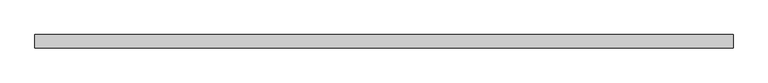
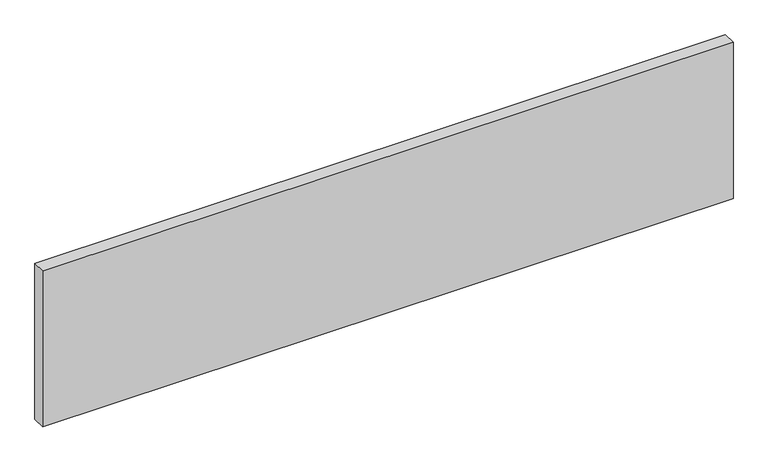
"""IFC4 building model written with IfcOpenShell, lengths in millimetres: proxy geometry, Plywood017 3466 : Plywood017 3466."""

import ifcopenshell
import ifcopenshell.guid

model = None  # the IFC model being written
_history = None  # IfcOwnerHistory: only IFC2X3 demands one
_inside = {}  # id of a spatial element -> (the spatial element, [elements in it])
_under = {}  # id of a project, library or spatial element -> (it, [spatial elements below it])
_declared = {}  # id of a project -> (the project, [libraries it declares])
_typed = {}  # id of a type object -> (the type object, [elements of that type])
_made_of = {}  # id of a material, layer set ... -> (it, [elements and type objects made of it])


def new_model(schema):
    """Start an empty IFC model of exactly this schema.

    Asked for "IFC4X3", IfcOpenShell would pick the latest addendum, in which some entities
    have other attributes; the version numbers below select the first issue.
    IFC2X3 requires an IfcOwnerHistory on every rooted entity: one is made here for all.
    """
    global model, _history
    if schema == "IFC4X3":
        model = ifcopenshell.file(schema_version=(4, 3, 0, 0))
    else:
        model = ifcopenshell.file(schema=schema)
    _inside.clear()
    _under.clear()
    _declared.clear()
    _typed.clear()
    _made_of.clear()
    _history = None
    if model.schema == "IFC2X3":
        org = make("IfcOrganization", Name="unknown")
        user = make(
            "IfcPersonAndOrganization",
            ThePerson=make("IfcPerson", FamilyName="unknown"),
            TheOrganization=org,
        )
        app = make(
            "IfcApplication",
            ApplicationDeveloper=org,
            Version="unknown",
            ApplicationFullName="unknown",
            ApplicationIdentifier="unknown",
        )
        _history = make(
            "IfcOwnerHistory",
            OwningUser=user,
            OwningApplication=app,
            ChangeAction="ADDED",
            CreationDate=0,
        )
    return model


def make(cls, **values):
    """One entity of the class cls with the attributes given. An attribute that is None is left unset."""
    return model.create_entity(
        cls, **{name: value for name, value in values.items() if value is not None}
    )


def rooted(cls, **values):
    """An entity with a GlobalId (a new one), such as an element, a storey or a relation."""
    return make(cls, GlobalId=ifcopenshell.guid.new(), OwnerHistory=_history, **values)


def si_unit(unit_type, name, prefix=None):
    """IfcSIUnit, for example si_unit("LENGTHUNIT", "METRE", prefix="MILLI")."""
    return make("IfcSIUnit", UnitType=unit_type, Prefix=prefix, Name=name)


def assignment(units):
    """IfcUnitAssignment: the units of a project."""
    return None if units is None else make("IfcUnitAssignment", Units=units)


def point(xyz):
    """IfcCartesianPoint."""
    return None if xyz is None else make("IfcCartesianPoint", Coordinates=xyz)


def direction(xyz):
    """IfcDirection."""
    return None if xyz is None else make("IfcDirection", DirectionRatios=xyz)


def frame(location, z_axis=None, x_axis=None):
    """IfcAxis2Placement3D, a coordinate frame: its origin and axes. An axis left out is left unset."""
    return make(
        "IfcAxis2Placement3D",
        Location=point(location),
        Axis=direction(z_axis),
        RefDirection=direction(x_axis),
    )


def origin():
    """The frame at (0, 0, 0) with its axes left unset."""
    return frame((0.0, 0.0, 0.0))


def place(relative_to, where):
    """IfcLocalPlacement: puts the frame where relative to a parent placement (None: the world)."""
    return make(
        "IfcLocalPlacement", PlacementRelTo=relative_to, RelativePlacement=where
    )


def context(
    kind, dimensions, precision=None, world=None, true_north=None, identifier=None
):
    """IfcGeometricRepresentationContext, for example the 3D "Model" context."""
    return make(
        "IfcGeometricRepresentationContext",
        ContextIdentifier=identifier,
        ContextType=kind,
        CoordinateSpaceDimension=dimensions,
        Precision=precision,
        WorldCoordinateSystem=world,
        TrueNorth=true_north,
    )


def project(units=None, contexts=None):
    """IfcProject with its units and contexts."""
    return rooted(
        "IfcProject",
        Name="project",
        RepresentationContexts=contexts,
        UnitsInContext=assignment(units),
    )


def spatial(cls, under=None, at=None, **own):
    """A site, building, storey or space (cls), placed at a placement, below another one or the project."""
    s = rooted(cls, ObjectPlacement=at, **own)
    if under is not None:
        _under.setdefault(under.id(), (under, []))[1].append(s)
    return s


def polyline(points):
    """IfcPolyline through the points."""
    return make("IfcPolyline", Points=[point(p) for p in points])


def outline(outer, holes=None, kind="AREA"):
    """IfcArbitraryClosedProfileDef: a profile drawn as a closed curve; with holes, ...WithVoids."""
    if holes is None:
        return make("IfcArbitraryClosedProfileDef", ProfileType=kind, OuterCurve=outer)
    return make(
        "IfcArbitraryProfileDefWithVoids",
        ProfileType=kind,
        OuterCurve=outer,
        InnerCurves=holes,
    )


def extrude(swept, where, along, depth):
    """IfcExtrudedAreaSolid: the profile swept, set in the frame where, extruded along a direction by depth."""
    return make(
        "IfcExtrudedAreaSolid",
        SweptArea=swept,
        Position=where,
        ExtrudedDirection=direction(along),
        Depth=depth,
    )


def shape(context_of_items, identifier, shape_type, items):
    """IfcShapeRepresentation: the items that make up one representation, for example the "Body"."""
    return make(
        "IfcShapeRepresentation",
        ContextOfItems=context_of_items,
        RepresentationIdentifier=identifier,
        RepresentationType=shape_type,
        Items=items,
    )


def source(mapping_origin, context_of_items, identifier, shape_type, items):
    """IfcRepresentationMap: a shape defined once, which mapped items show again and again."""
    return make(
        "IfcRepresentationMap",
        MappingOrigin=mapping_origin,
        MappedRepresentation=shape(context_of_items, identifier, shape_type, items),
    )


def transform(
    local_origin,
    x_axis=None,
    y_axis=None,
    z_axis=None,
    scale=None,
    scale2=None,
    scale3=None,
    uniform=True,
):
    """IfcCartesianTransformationOperator3D, or its non-uniform kind. x_axis, y_axis, z_axis: its Axis1, 2, 3."""
    if uniform:
        return make(
            "IfcCartesianTransformationOperator3D",
            Axis1=direction(x_axis),
            Axis2=direction(y_axis),
            LocalOrigin=point(local_origin),
            Scale=scale,
            Axis3=direction(z_axis),
        )
    return make(
        "IfcCartesianTransformationOperator3DnonUniform",
        Axis1=direction(x_axis),
        Axis2=direction(y_axis),
        LocalOrigin=point(local_origin),
        Scale=scale,
        Axis3=direction(z_axis),
        Scale2=scale2,
        Scale3=scale3,
    )


def mapped(mapping_source, mapping_target):
    """IfcMappedItem: shows the shape of a source again, moved by a transform."""
    return make(
        "IfcMappedItem", MappingSource=mapping_source, MappingTarget=mapping_target
    )


def made_of(thing, what):
    """Note that an element or type object is made of a material, layer set ...; save() writes the relation."""
    if what is not None:
        _made_of.setdefault(what.id(), (what, []))[1].append(thing)
    return thing


def element(
    cls,
    number,
    at=None,
    inside=None,
    cuts=None,
    type_object=None,
    material=None,
    context=None,
    identifier="Body",
    shape_type=None,
    held_by="IfcProductDefinitionShape",
    body=None,
    shapes=None,
    **own,
):
    """One element of the class cls, such as IfcWall. Its Tag is "e" and its number.

    at: its placement. inside: the storey or other place that contains it. cuts: it is an
    opening in that element (IfcRelVoidsElement). A single representation is given by context,
    identifier, shape_type and body (its items); several are given by shapes. held_by: the class
    of the entity that holds the representations. save() writes the other relations.
    """
    e = rooted(cls, Tag="e%d" % number, ObjectPlacement=at, **own)
    if body is not None:
        shapes = [shape(context, identifier, shape_type, body)]
    if shapes is not None:
        e.Representation = make(held_by, Representations=shapes)
    if inside is not None:
        _inside.setdefault(inside.id(), (inside, []))[1].append(e)
    if cuts is not None:
        rooted(
            "IfcRelVoidsElement", RelatingBuildingElement=cuts, RelatedOpeningElement=e
        )
    if type_object is not None:
        _typed.setdefault(type_object.id(), (type_object, []))[1].append(e)
    return made_of(e, material)


def aggregate(whole, parts):
    """IfcRelAggregates: a whole, such as a stair, and the parts it consists of."""
    return rooted("IfcRelAggregates", RelatingObject=whole, RelatedObjects=parts)


def save(model, path):
    """Write the relations noted so far, then the file.

    IfcRelAggregates (storeys below a building ...), IfcRelContainedInSpatialStructure (elements
    in a storey), IfcRelDefinesByType, IfcRelAssociatesMaterial and IfcRelDeclares: one each for
    every whole, place, type object, material and project.
    """
    for whole, parts in _under.values():
        aggregate(whole, parts)
    for where, things in _inside.values():
        rooted(
            "IfcRelContainedInSpatialStructure",
            RelatedElements=things,
            RelatingStructure=where,
        )
    for kind, things in _typed.values():
        rooted("IfcRelDefinesByType", RelatedObjects=things, RelatingType=kind)
    for what, things in _made_of.values():
        rooted("IfcRelAssociatesMaterial", RelatedObjects=things, RelatingMaterial=what)
    for by, libraries in _declared.values():
        rooted("IfcRelDeclares", RelatingContext=by, RelatedDefinitions=libraries)
    model.write(path)


def generic_models_d8a1cbeb(model_context):
    return source(origin(), model_context, "Body", "SweptSolid", [
        extrude(outline(polyline([(3694.2883192, 10765.3875834), (3694.2883192, 10803.4875834), (5694.2883192, 10803.4875834), (5694.2883192, 10765.3875834), (3694.2883192, 10765.3875834)])), frame((0.0, 0.0, 43499.4557108), z_axis=(0.0, 0.0, 1.0), x_axis=(1.0, 0.0, 0.0)), (0.0, 0.0, 1.0), 478.6164062),
    ])


if __name__ == "__main__":
    model = new_model("IFC4")
    model_context = context("Model", 3, world=origin())
    ifc_project = project(units=[si_unit("LENGTHUNIT", "METRE", prefix="MILLI")], contexts=[model_context])
    site = spatial("IfcSite", under=ifc_project)
    building = spatial("IfcBuilding", under=site)
    placement = place(None, origin())
    generic_models_shape = generic_models_d8a1cbeb(model_context)
    element("IfcBuildingElementProxy", 1, Name="Plywood017 3466 : Plywood017 3466", ObjectType="Plywood017 3466 : Plywood017 3466", at=placement, inside=building, context=model_context, shape_type="MappedRepresentation", body=[
        mapped(generic_models_shape, transform((0.0, 0.0, 0.0), x_axis=(1.0, 0.0, 0.0), y_axis=(0.0, 1.0, 0.0), z_axis=(0.0, 0.0, 1.0))),
    ])
    save(model, "model.ifc")

# Revit data of these elements
# Type "Plywood017 3466 : Plywood017 3466"
#   NameOverride = "Plywood017"
# Element 1 (IfcBuildingElementProxy, "Plywood017 3466 : Plywood017 3466")
#   Materials on its faces: "CDX PLYWOOD - SEE STRUCTURAL DWGS"
# Materials
#   "CDX PLYWOOD - SEE STRUCTURAL DWGS": class "Unassigned", colour RGB 177 130 114, transparency 0, Cost = 0
